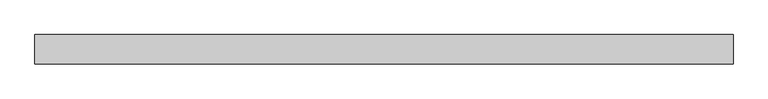
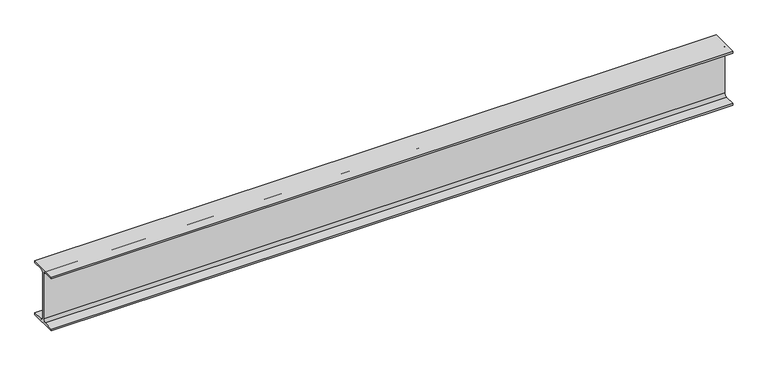
"""IFC4 building model written with IfcOpenShell, lengths in millimetres: beam geometry, 0912_Steel Framing_H-KSD3502 : H_SB_ASB_H-250x125x6x9."""

import ifcopenshell
import ifcopenshell.guid

model = None  # the IFC model being written
_history = None  # IfcOwnerHistory: only IFC2X3 demands one
_inside = {}  # id of a spatial element -> (the spatial element, [elements in it])
_under = {}  # id of a project, library or spatial element -> (it, [spatial elements below it])
_declared = {}  # id of a project -> (the project, [libraries it declares])
_typed = {}  # id of a type object -> (the type object, [elements of that type])
_made_of = {}  # id of a material, layer set ... -> (it, [elements and type objects made of it])


def new_model(schema):
    """Start an empty IFC model of exactly this schema.

    Asked for "IFC4X3", IfcOpenShell would pick the latest addendum, in which some entities
    have other attributes; the version numbers below select the first issue.
    IFC2X3 requires an IfcOwnerHistory on every rooted entity: one is made here for all.
    """
    global model, _history
    if schema == "IFC4X3":
        model = ifcopenshell.file(schema_version=(4, 3, 0, 0))
    else:
        model = ifcopenshell.file(schema=schema)
    _inside.clear()
    _under.clear()
    _declared.clear()
    _typed.clear()
    _made_of.clear()
    _history = None
    if model.schema == "IFC2X3":
        org = make("IfcOrganization", Name="unknown")
        user = make(
            "IfcPersonAndOrganization",
            ThePerson=make("IfcPerson", FamilyName="unknown"),
            TheOrganization=org,
        )
        app = make(
            "IfcApplication",
            ApplicationDeveloper=org,
            Version="unknown",
            ApplicationFullName="unknown",
            ApplicationIdentifier="unknown",
        )
        _history = make(
            "IfcOwnerHistory",
            OwningUser=user,
            OwningApplication=app,
            ChangeAction="ADDED",
            CreationDate=0,
        )
    return model


def make(cls, **values):
    """One entity of the class cls with the attributes given. An attribute that is None is left unset."""
    return model.create_entity(
        cls, **{name: value for name, value in values.items() if value is not None}
    )


def rooted(cls, **values):
    """An entity with a GlobalId (a new one), such as an element, a storey or a relation."""
    return make(cls, GlobalId=ifcopenshell.guid.new(), OwnerHistory=_history, **values)


def si_unit(unit_type, name, prefix=None):
    """IfcSIUnit, for example si_unit("LENGTHUNIT", "METRE", prefix="MILLI")."""
    return make("IfcSIUnit", UnitType=unit_type, Prefix=prefix, Name=name)


def assignment(units):
    """IfcUnitAssignment: the units of a project."""
    return None if units is None else make("IfcUnitAssignment", Units=units)


def point(xyz):
    """IfcCartesianPoint."""
    return None if xyz is None else make("IfcCartesianPoint", Coordinates=xyz)


def direction(xyz):
    """IfcDirection."""
    return None if xyz is None else make("IfcDirection", DirectionRatios=xyz)


def frame(location, z_axis=None, x_axis=None):
    """IfcAxis2Placement3D, a coordinate frame: its origin and axes. An axis left out is left unset."""
    return make(
        "IfcAxis2Placement3D",
        Location=point(location),
        Axis=direction(z_axis),
        RefDirection=direction(x_axis),
    )


def frame_2d(location, x_axis=None):
    """IfcAxis2Placement2D, a coordinate frame in the plane: its origin and x axis."""
    return make(
        "IfcAxis2Placement2D", Location=point(location), RefDirection=direction(x_axis)
    )


def origin():
    """The frame at (0, 0, 0) with its axes left unset."""
    return frame((0.0, 0.0, 0.0))


def place(relative_to, where):
    """IfcLocalPlacement: puts the frame where relative to a parent placement (None: the world)."""
    return make(
        "IfcLocalPlacement", PlacementRelTo=relative_to, RelativePlacement=where
    )


def context(
    kind, dimensions, precision=None, world=None, true_north=None, identifier=None
):
    """IfcGeometricRepresentationContext, for example the 3D "Model" context."""
    return make(
        "IfcGeometricRepresentationContext",
        ContextIdentifier=identifier,
        ContextType=kind,
        CoordinateSpaceDimension=dimensions,
        Precision=precision,
        WorldCoordinateSystem=world,
        TrueNorth=true_north,
    )


def project(units=None, contexts=None):
    """IfcProject with its units and contexts."""
    return rooted(
        "IfcProject",
        Name="project",
        RepresentationContexts=contexts,
        UnitsInContext=assignment(units),
    )


def spatial(cls, under=None, at=None, **own):
    """A site, building, storey or space (cls), placed at a placement, below another one or the project."""
    s = rooted(cls, ObjectPlacement=at, **own)
    if under is not None:
        _under.setdefault(under.id(), (under, []))[1].append(s)
    return s


def polyline(points):
    """IfcPolyline through the points."""
    return make("IfcPolyline", Points=[point(p) for p in points])


def circle_curve(where, radius):
    """IfcCircle in the frame where."""
    return make("IfcCircle", Position=where, Radius=radius)


def trimmed(basis, trim1, trim2, sense, master):
    """IfcTrimmedCurve: the piece of a basis curve between two trims."""
    return make(
        "IfcTrimmedCurve",
        BasisCurve=basis,
        Trim1=trim1,
        Trim2=trim2,
        SenseAgreement=sense,
        MasterRepresentation=master,
    )


def segment(curve, same_sense, transition):
    """IfcCompositeCurveSegment."""
    return make(
        "IfcCompositeCurveSegment",
        Transition=transition,
        SameSense=same_sense,
        ParentCurve=curve,
    )


def composite_curve(segments, self_intersect=None):
    """IfcCompositeCurve: segments joined end to end."""
    return make("IfcCompositeCurve", Segments=segments, SelfIntersect=self_intersect)


def outline(outer, holes=None, kind="AREA"):
    """IfcArbitraryClosedProfileDef: a profile drawn as a closed curve; with holes, ...WithVoids."""
    if holes is None:
        return make("IfcArbitraryClosedProfileDef", ProfileType=kind, OuterCurve=outer)
    return make(
        "IfcArbitraryProfileDefWithVoids",
        ProfileType=kind,
        OuterCurve=outer,
        InnerCurves=holes,
    )


def extrude(swept, where, along, depth):
    """IfcExtrudedAreaSolid: the profile swept, set in the frame where, extruded along a direction by depth."""
    return make(
        "IfcExtrudedAreaSolid",
        SweptArea=swept,
        Position=where,
        ExtrudedDirection=direction(along),
        Depth=depth,
    )


def shape(context_of_items, identifier, shape_type, items):
    """IfcShapeRepresentation: the items that make up one representation, for example the "Body"."""
    return make(
        "IfcShapeRepresentation",
        ContextOfItems=context_of_items,
        RepresentationIdentifier=identifier,
        RepresentationType=shape_type,
        Items=items,
    )


def source(mapping_origin, context_of_items, identifier, shape_type, items):
    """IfcRepresentationMap: a shape defined once, which mapped items show again and again."""
    return make(
        "IfcRepresentationMap",
        MappingOrigin=mapping_origin,
        MappedRepresentation=shape(context_of_items, identifier, shape_type, items),
    )


def transform(
    local_origin,
    x_axis=None,
    y_axis=None,
    z_axis=None,
    scale=None,
    scale2=None,
    scale3=None,
    uniform=True,
):
    """IfcCartesianTransformationOperator3D, or its non-uniform kind. x_axis, y_axis, z_axis: its Axis1, 2, 3."""
    if uniform:
        return make(
            "IfcCartesianTransformationOperator3D",
            Axis1=direction(x_axis),
            Axis2=direction(y_axis),
            LocalOrigin=point(local_origin),
            Scale=scale,
            Axis3=direction(z_axis),
        )
    return make(
        "IfcCartesianTransformationOperator3DnonUniform",
        Axis1=direction(x_axis),
        Axis2=direction(y_axis),
        LocalOrigin=point(local_origin),
        Scale=scale,
        Axis3=direction(z_axis),
        Scale2=scale2,
        Scale3=scale3,
    )


def mapped(mapping_source, mapping_target):
    """IfcMappedItem: shows the shape of a source again, moved by a transform."""
    return make(
        "IfcMappedItem", MappingSource=mapping_source, MappingTarget=mapping_target
    )


def made_of(thing, what):
    """Note that an element or type object is made of a material, layer set ...; save() writes the relation."""
    if what is not None:
        _made_of.setdefault(what.id(), (what, []))[1].append(thing)
    return thing


def element(
    cls,
    number,
    at=None,
    inside=None,
    cuts=None,
    type_object=None,
    material=None,
    context=None,
    identifier="Body",
    shape_type=None,
    held_by="IfcProductDefinitionShape",
    body=None,
    shapes=None,
    **own,
):
    """One element of the class cls, such as IfcWall. Its Tag is "e" and its number.

    at: its placement. inside: the storey or other place that contains it. cuts: it is an
    opening in that element (IfcRelVoidsElement). A single representation is given by context,
    identifier, shape_type and body (its items); several are given by shapes. held_by: the class
    of the entity that holds the representations. save() writes the other relations.
    """
    e = rooted(cls, Tag="e%d" % number, ObjectPlacement=at, **own)
    if body is not None:
        shapes = [shape(context, identifier, shape_type, body)]
    if shapes is not None:
        e.Representation = make(held_by, Representations=shapes)
    if inside is not None:
        _inside.setdefault(inside.id(), (inside, []))[1].append(e)
    if cuts is not None:
        rooted(
            "IfcRelVoidsElement", RelatingBuildingElement=cuts, RelatedOpeningElement=e
        )
    if type_object is not None:
        _typed.setdefault(type_object.id(), (type_object, []))[1].append(e)
    return made_of(e, material)


def aggregate(whole, parts):
    """IfcRelAggregates: a whole, such as a stair, and the parts it consists of."""
    return rooted("IfcRelAggregates", RelatingObject=whole, RelatedObjects=parts)


def save(model, path):
    """Write the relations noted so far, then the file.

    IfcRelAggregates (storeys below a building ...), IfcRelContainedInSpatialStructure (elements
    in a storey), IfcRelDefinesByType, IfcRelAssociatesMaterial and IfcRelDeclares: one each for
    every whole, place, type object, material and project.
    """
    for whole, parts in _under.values():
        aggregate(whole, parts)
    for where, things in _inside.values():
        rooted(
            "IfcRelContainedInSpatialStructure",
            RelatedElements=things,
            RelatingStructure=where,
        )
    for kind, things in _typed.values():
        rooted("IfcRelDefinesByType", RelatedObjects=things, RelatingType=kind)
    for what, things in _made_of.values():
        rooted("IfcRelAssociatesMaterial", RelatedObjects=things, RelatingMaterial=what)
    for by, libraries in _declared.values():
        rooted("IfcRelDeclares", RelatingContext=by, RelatedDefinitions=libraries)
    model.write(path)


def beam_64758b51(model_context):
    return source(origin(), model_context, "Body", "SweptSolid", [
        extrude(outline(composite_curve([segment(polyline([(62.5, -116.0), (62.5, -125.0), (-62.5, -125.0), (-62.5, -116.0), (-15.0, -116.0)]), True, "CONTINUOUS"), segment(trimmed(circle_curve(frame_2d((-15.0, -104.0)), 12.0), [point((-15.0, -116.0))], [point((-3.0, -104.0))], True, "CARTESIAN"), True, "CONTINUOUS"), segment(polyline([(-3.0, -104.0), (-3.0, 104.0)]), True, "CONTINUOUS"), segment(trimmed(circle_curve(frame_2d((-15.0, 104.0)), 12.0), [point((-3.0, 104.0))], [point((-15.0, 116.0))], True, "CARTESIAN"), True, "CONTINUOUS"), segment(polyline([(-15.0, 116.0), (-62.5, 116.0), (-62.5, 125.0), (62.5, 125.0), (62.5, 116.0), (15.0, 116.0)]), True, "CONTINUOUS"), segment(trimmed(circle_curve(frame_2d((15.0, 104.0)), 12.0), [point((15.0, 116.0))], [point((3.0, 104.0))], True, "CARTESIAN"), True, "CONTINUOUS"), segment(polyline([(3.0, 104.0), (3.0, -104.0)]), True, "CONTINUOUS"), segment(trimmed(circle_curve(frame_2d((15.0, -104.0)), 12.0), [point((3.0, -104.0))], [point((15.0, -116.0))], True, "CARTESIAN"), True, "CONTINUOUS"), segment(polyline([(15.0, -116.0), (62.5, -116.0)]), True, "CONTINUOUS")], self_intersect=False)), frame((-1493.3, 0.0, 0.0), z_axis=(1.0, 0.0, 0.0), x_axis=(0.0, 1.0, 0.0)), (0.0, 0.0, 1.0), 2987.8360727),
    ])


if __name__ == "__main__":
    model = new_model("IFC4")
    model_context = context("Model", 3, world=origin())
    ifc_project = project(units=[si_unit("LENGTHUNIT", "METRE", prefix="MILLI")], contexts=[model_context])
    site = spatial("IfcSite", under=ifc_project)
    building = spatial("IfcBuilding", under=site)
    placement = place(None, origin())
    beam_shape = beam_64758b51(model_context)
    element("IfcBeam", 1, ObjectType="0912_Steel Framing_H-KSD3502 : H_SB_ASB_H-250x125x6x9", at=placement, inside=building, context=model_context, shape_type="MappedRepresentation", body=[
        mapped(beam_shape, transform((0.0, 0.0, 0.0), x_axis=(1.0, 0.0, 0.0), y_axis=(0.0, 1.0, 0.0), z_axis=(0.0, 0.0, 1.0))),
    ])
    save(model, "model.ifc")

# Revit data of these elements
# Type "0912_Steel Framing_H-KSD3502 : H_SB_ASB_H-250x125x6x9"
#   H_WM Code_1 = "S01AA003-00001 | Main Steel Structure Fabrication Work | Shelter/Building | Light Steel - Standard (30KG/M>Weight) | Material: (   )"
#   H_WM Code_2 = "S03AA029-00001 | Main Steel Structure Erection Work | Shelter/Building | Light Steel (30KG/M>Weight) | Material: (   )"
#   H_WM Code_3 = "S01AA010-00001 | Main Steel Structure Fabrication Work | Shelter/Building | Steel Painting/Coating | for Non-Fireproofed Steel Surface, Surface Preparation, Primer, Second & Final Coat | Material: (   )"
#   H_Q'ty Cal Type Tag = "SB-Q2"
#   Width = 12.5 cm
#   Web Thickness = 0.6 cm
#   Web Fillet = 1.2 cm
#   Warping Constant = 42539.8 cm⁶
#   W = 0
#   Torsional Moment of Inertia = 7.8102 cm⁴
#   Section Area = 37.66 cm²
#   Plastic Modulus weak axis = 73.1 cm³
#   Plastic Modulus strong axis = 366.0 cm³
#   Perimeter = 0.97 m²/m
#   Nominal Weight = 29.60 kgf/m
#   Moment of Inertia weak axis = 294.00 cm⁴
#   Moment of Inertia strong axis = 4050.00 cm⁴
#   Height = 25.0 cm
#   Flange Thickness = 0.9 cm
#   Elastic Modulus weak axis = 47.0 cm³
#   Elastic Modulus strong axis = 324.0 cm³
#   Centroid Vertical = 12.5 cm
#   Centroid Horizontal = 6.25 cm
#   Ix = 40500000
#   Length [instance default] = 1.5240 m
#   Zx = 366000
#   b = 0.1250 m
#   h = 0.2500 m
#   r = 0.0120 m
#   s = 0.0060 m
#   t = 0.0090 m
#   A = 0.003766 m²
#   Structural Material [instance default] = Steel, 45-345
#   Assembly Code = ""
# Element 1 (IfcBeam, "0912_Steel Framing_H-KSD3502 : H_SB_ASB_H-250x125x6x9")
#   Structural Material = none
# Materials
#   "Steel, 45-345": class "Metal", colour RGB 189 187 185, transparency 0, Description = "Steel 345 MPa", Cost = 0
